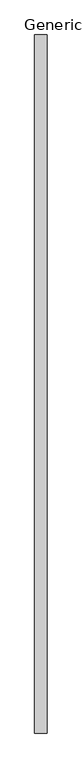
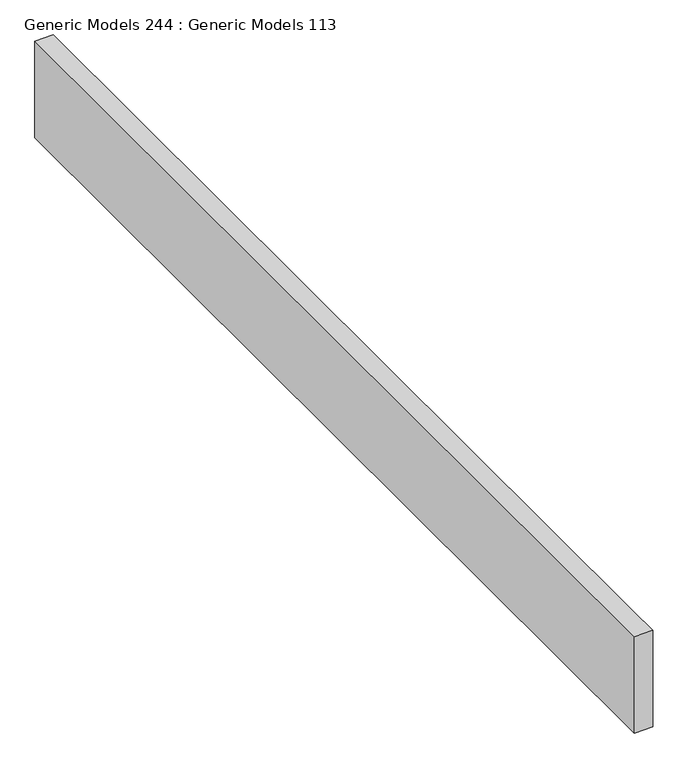
"""IFC4 building model written with IfcOpenShell, lengths in millimetres: proxy geometry, Generic Models 244 : Generic Models 113."""

from ifc_helpers import new_model, si_unit, origin, place, context, project, spatial, faceted_brep, source, transform, mapped, element, save


def generic_models_244_generic_models_113_daa3e339(model_context):
    return source(origin(), model_context, "Body", "Brep", [
        faceted_brep([(31888.1210525, 39454.8946413, 266245.6765953), (32090.9670184, 39454.8946413, 266245.6765953), (32090.9670184, 39454.8946413, 265128.375), (31888.1210525, 39454.8946413, 265128.375), (31888.1210525, 28080.2169475, 266245.6765953), (31888.1210525, 28080.2169475, 265128.375), (32090.9670184, 28080.2169475, 265128.375), (32090.9670184, 28080.2169475, 266245.6765953), (32090.9670184, 28439.2747112, 266245.6765953)], [[[0, 1, 2, 3]], [[4, 5, 6, 7]], [[1, 0, 4, 7, 8]], [[2, 1, 8, 7, 6]], [[3, 2, 6, 5]], [[0, 3, 5, 4]]]),
    ])


if __name__ == "__main__":
    model = new_model("IFC4")
    model_context = context("Model", 3, world=origin())
    ifc_project = project(units=[si_unit("LENGTHUNIT", "METRE", prefix="MILLI")], contexts=[model_context])
    site = spatial("IfcSite", under=ifc_project)
    building = spatial("IfcBuilding", under=site)
    placement = place(None, origin())
    generic_models_244_generic_models_113_shape = generic_models_244_generic_models_113_daa3e339(model_context)
    element("IfcBuildingElementProxy", 1, Name="Generic Models 244 : Generic Models 113", ObjectType="Generic Models 244 : Generic Models 113", at=placement, inside=building, context=model_context, shape_type="MappedRepresentation", body=[
        mapped(generic_models_244_generic_models_113_shape, transform((0.0, 0.0, 0.0), x_axis=(1.0, 0.0, 0.0), y_axis=(0.0, 1.0, 0.0), z_axis=(0.0, 0.0, 1.0))),
    ])
    save(model, "model.ifc")

# Revit data of these elements
# Element 1 (IfcBuildingElementProxy, "Generic Models 244 : Generic Models 113")
#   Materials on its faces: "EXISTING CONCRETE FOUNDATION WALL"
# Materials
#   "EXISTING CONCRETE FOUNDATION WALL": class "Concrete", colour RGB 192 192 192, transparency 0, Description = "Cast-in-place concrete", Cost = 0
